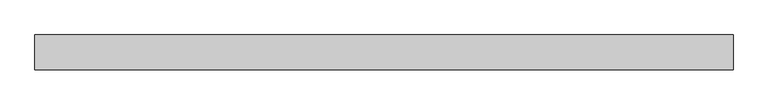
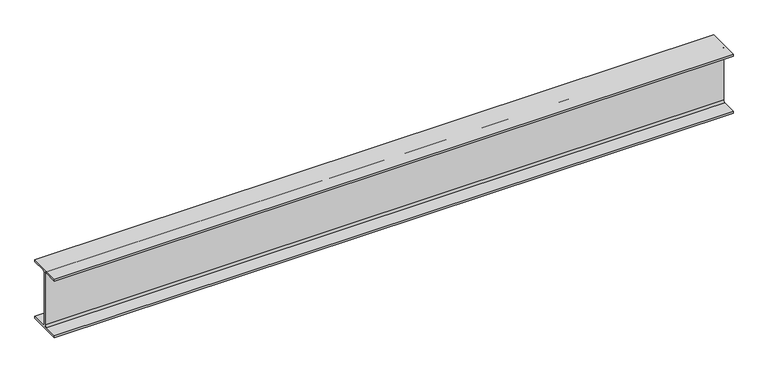
"""IFC4 building model written with IfcOpenShell, lengths in millimetres: beam geometry, Old_Steel Beam_H-KSD3502 : H_SB_ASB_H-200×200x8x12."""

from ifc_helpers import new_model, si_unit, point, frame, frame_2d, origin, place, context, project, spatial, polyline, circle_curve, trimmed, segment, composite_curve, outline, extrude, source, transform, mapped, element, save


def beam_bca2621f(model_context):
    return source(origin(), model_context, "Body", "SweptSolid", [
        extrude(outline(composite_curve([segment(polyline([(82.5, -141.5), (82.5, -151.7), (-82.5, -151.7), (-82.5, -141.5), (-11.9, -141.5)]), True, "CONTINUOUS"), segment(trimmed(circle_curve(frame_2d((-11.9, -132.6)), 8.9), [point((-11.9, -141.5))], [point((-3.0, -132.6))], True, "CARTESIAN"), True, "CONTINUOUS"), segment(polyline([(-3.0, -132.6), (-3.0, 132.6)]), True, "CONTINUOUS"), segment(trimmed(circle_curve(frame_2d((-11.9, 132.6)), 8.9), [point((-3.0, 132.6))], [point((-11.9, 141.5))], True, "CARTESIAN"), True, "CONTINUOUS"), segment(polyline([(-11.9, 141.5), (-82.5, 141.5), (-82.5, 151.7), (82.5, 151.7), (82.5, 141.5), (11.9, 141.5)]), True, "CONTINUOUS"), segment(trimmed(circle_curve(frame_2d((11.9, 132.6)), 8.9), [point((11.9, 141.5))], [point((3.0, 132.6))], True, "CARTESIAN"), True, "CONTINUOUS"), segment(polyline([(3.0, 132.6), (3.0, -132.6)]), True, "CONTINUOUS"), segment(trimmed(circle_curve(frame_2d((11.9, -132.6)), 8.9), [point((3.0, -132.6))], [point((11.9, -141.5))], True, "CARTESIAN"), True, "CONTINUOUS"), segment(polyline([(11.9, -141.5), (82.5, -141.5)]), True, "CONTINUOUS")], self_intersect=False)), frame((-1594.31566, 0.0, 0.0), z_axis=(1.0, 0.0, 0.0), x_axis=(0.0, 1.0, 0.0)), (0.0, 0.0, 1.0), 3316.0486402),
    ])


if __name__ == "__main__":
    model = new_model("IFC4")
    model_context = context("Model", 3, world=origin())
    ifc_project = project(units=[si_unit("LENGTHUNIT", "METRE", prefix="MILLI")], contexts=[model_context])
    site = spatial("IfcSite", under=ifc_project)
    building = spatial("IfcBuilding", under=site)
    placement = place(None, origin())
    beam_shape = beam_bca2621f(model_context)
    element("IfcBeam", 1, ObjectType="Old_Steel Beam_H-KSD3502 : H_SB_ASB_H-200×200x8x12", at=placement, inside=building, context=model_context, shape_type="MappedRepresentation", body=[
        mapped(beam_shape, transform((0.0, 0.0, 0.0), x_axis=(1.0, 0.0, 0.0), y_axis=(0.0, 1.0, 0.0), z_axis=(0.0, 0.0, 1.0))),
    ])
    save(model, "model.ifc")

# Revit data of these elements
# Type "Old_Steel Beam_H-KSD3502 : H_SB_ASB_H-200×200x8x12"
#   Width = 20.0 cm
#   Web Thickness = 0.8 cm
#   Web Fillet = 1.3 cm
#   Warping Constant = 141376.0 cm⁶
#   Torsional Moment of Inertia = 26.2485 cm⁴
#   Torsional Modulus = 1.0 cm³
#   Section Area = 63.53 cm²
#   Plastic Modulus weak axis = 244.0 cm³
#   Plastic Modulus strong axis = 525.0 cm³
#   Perimeter = 1.16 m²/m
#   Nominal Weight = 49.90 kgf/m
#   Moment of Inertia weak axis = 1600.00 cm⁴
#   Moment of Inertia strong axis = 4720.00 cm⁴
#   Height = 20.0 cm
#   Flange Thickness = 1.2 cm
#   Elastic Modulus weak axis = 160.0 cm³
#   Elastic Modulus strong axis = 472.0 cm³
#   Centroid Vertical = 10.0 cm
#   Centroid Horizontal = 10.0 cm
#   Length [instance default] = 1.5240 m
#   Structural Material [instance default] = Steel, 45-345
#   Assembly Code = ""
# Element 1 (IfcBeam, "Old_Steel Beam_H-KSD3502 : H_SB_ASB_H-200×200x8x12")
#   Structural Material = none
# Materials
#   "Steel, 45-345": class "Metal", colour RGB 189 187 185, transparency 0, Description = "Steel 345 MPa", Cost = 0
